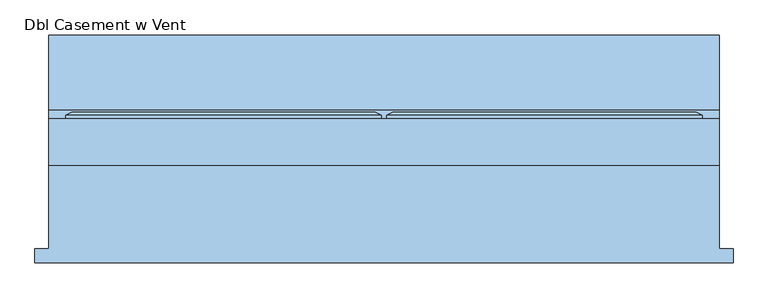
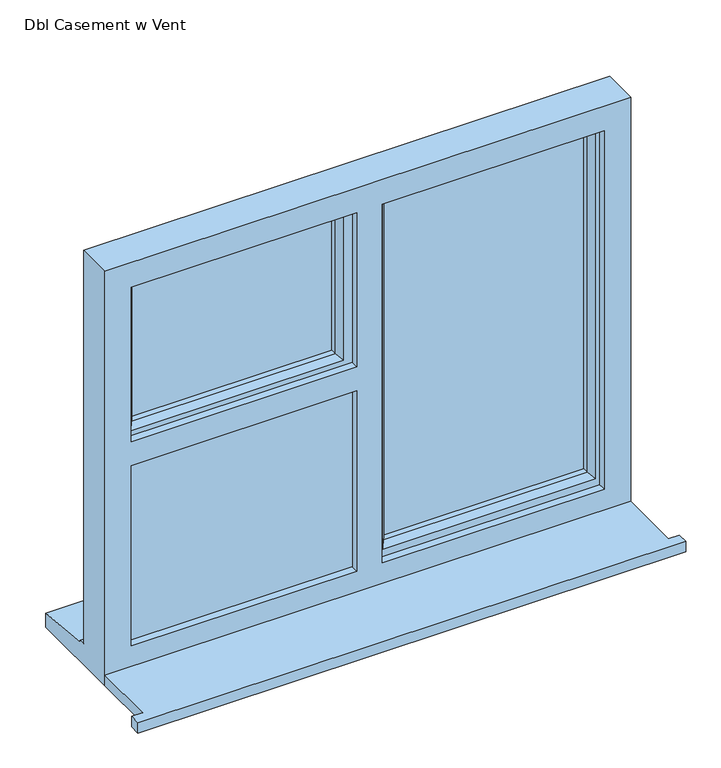
"""IFC4 building model written with IfcOpenShell, lengths in millimetres: window geometry, Dbl Casement w Vent : Doublel Casement with Vent 1200w x 1000h."""

import ifcopenshell
import ifcopenshell.guid

model = None  # the IFC model being written
_history = None  # IfcOwnerHistory: only IFC2X3 demands one
_inside = {}  # id of a spatial element -> (the spatial element, [elements in it])
_under = {}  # id of a project, library or spatial element -> (it, [spatial elements below it])
_declared = {}  # id of a project -> (the project, [libraries it declares])
_typed = {}  # id of a type object -> (the type object, [elements of that type])
_made_of = {}  # id of a material, layer set ... -> (it, [elements and type objects made of it])


def new_model(schema):
    """Start an empty IFC model of exactly this schema.

    Asked for "IFC4X3", IfcOpenShell would pick the latest addendum, in which some entities
    have other attributes; the version numbers below select the first issue.
    IFC2X3 requires an IfcOwnerHistory on every rooted entity: one is made here for all.
    """
    global model, _history
    if schema == "IFC4X3":
        model = ifcopenshell.file(schema_version=(4, 3, 0, 0))
    else:
        model = ifcopenshell.file(schema=schema)
    _inside.clear()
    _under.clear()
    _declared.clear()
    _typed.clear()
    _made_of.clear()
    _history = None
    if model.schema == "IFC2X3":
        org = make("IfcOrganization", Name="unknown")
        user = make(
            "IfcPersonAndOrganization",
            ThePerson=make("IfcPerson", FamilyName="unknown"),
            TheOrganization=org,
        )
        app = make(
            "IfcApplication",
            ApplicationDeveloper=org,
            Version="unknown",
            ApplicationFullName="unknown",
            ApplicationIdentifier="unknown",
        )
        _history = make(
            "IfcOwnerHistory",
            OwningUser=user,
            OwningApplication=app,
            ChangeAction="ADDED",
            CreationDate=0,
        )
    return model


def make(cls, **values):
    """One entity of the class cls with the attributes given. An attribute that is None is left unset."""
    return model.create_entity(
        cls, **{name: value for name, value in values.items() if value is not None}
    )


def rooted(cls, **values):
    """An entity with a GlobalId (a new one), such as an element, a storey or a relation."""
    return make(cls, GlobalId=ifcopenshell.guid.new(), OwnerHistory=_history, **values)


def si_unit(unit_type, name, prefix=None):
    """IfcSIUnit, for example si_unit("LENGTHUNIT", "METRE", prefix="MILLI")."""
    return make("IfcSIUnit", UnitType=unit_type, Prefix=prefix, Name=name)


def assignment(units):
    """IfcUnitAssignment: the units of a project."""
    return None if units is None else make("IfcUnitAssignment", Units=units)


def point(xyz):
    """IfcCartesianPoint."""
    return None if xyz is None else make("IfcCartesianPoint", Coordinates=xyz)


def direction(xyz):
    """IfcDirection."""
    return None if xyz is None else make("IfcDirection", DirectionRatios=xyz)


def frame(location, z_axis=None, x_axis=None):
    """IfcAxis2Placement3D, a coordinate frame: its origin and axes. An axis left out is left unset."""
    return make(
        "IfcAxis2Placement3D",
        Location=point(location),
        Axis=direction(z_axis),
        RefDirection=direction(x_axis),
    )


def origin():
    """The frame at (0, 0, 0) with its axes left unset."""
    return frame((0.0, 0.0, 0.0))


def place(relative_to, where):
    """IfcLocalPlacement: puts the frame where relative to a parent placement (None: the world)."""
    return make(
        "IfcLocalPlacement", PlacementRelTo=relative_to, RelativePlacement=where
    )


def context(
    kind, dimensions, precision=None, world=None, true_north=None, identifier=None
):
    """IfcGeometricRepresentationContext, for example the 3D "Model" context."""
    return make(
        "IfcGeometricRepresentationContext",
        ContextIdentifier=identifier,
        ContextType=kind,
        CoordinateSpaceDimension=dimensions,
        Precision=precision,
        WorldCoordinateSystem=world,
        TrueNorth=true_north,
    )


def project(units=None, contexts=None):
    """IfcProject with its units and contexts."""
    return rooted(
        "IfcProject",
        Name="project",
        RepresentationContexts=contexts,
        UnitsInContext=assignment(units),
    )


def spatial(cls, under=None, at=None, **own):
    """A site, building, storey or space (cls), placed at a placement, below another one or the project."""
    s = rooted(cls, ObjectPlacement=at, **own)
    if under is not None:
        _under.setdefault(under.id(), (under, []))[1].append(s)
    return s


def polyline(points):
    """IfcPolyline through the points."""
    return make("IfcPolyline", Points=[point(p) for p in points])


def outline(outer, holes=None, kind="AREA"):
    """IfcArbitraryClosedProfileDef: a profile drawn as a closed curve; with holes, ...WithVoids."""
    if holes is None:
        return make("IfcArbitraryClosedProfileDef", ProfileType=kind, OuterCurve=outer)
    return make(
        "IfcArbitraryProfileDefWithVoids",
        ProfileType=kind,
        OuterCurve=outer,
        InnerCurves=holes,
    )


def extrude(swept, where, along, depth):
    """IfcExtrudedAreaSolid: the profile swept, set in the frame where, extruded along a direction by depth."""
    return make(
        "IfcExtrudedAreaSolid",
        SweptArea=swept,
        Position=where,
        ExtrudedDirection=direction(along),
        Depth=depth,
    )


def faces_of(points, faces, orient=None, outer=None):
    """IfcFace entities. A face is a list of loops; a loop is a list of indices into points, from 0.

    orient and outer hold one flag for each loop. By default every Orientation is true, the
    first loop of a face is its IfcFaceOuterBound and the others are IfcFaceBound.
    """
    made = []
    for i, loops in enumerate(faces):
        bounds = []
        for j, loop in enumerate(loops):
            is_outer = j == 0 if outer is None else outer[i][j]
            bounds.append(
                make(
                    "IfcFaceOuterBound" if is_outer else "IfcFaceBound",
                    Bound=make("IfcPolyLoop", Polygon=[points[k] for k in loop]),
                    Orientation=True if orient is None else orient[i][j],
                )
            )
        made.append(make("IfcFace", Bounds=bounds))
    return made


def faceted_brep(points, faces, orient=None, outer=None, voids=None):
    """IfcFacetedBrep: a solid bounded by flat faces; with voids (closed shells), ...WithVoids."""
    shared = [point(p) for p in points]
    hull = make("IfcClosedShell", CfsFaces=faces_of(shared, faces, orient, outer))
    if voids is None:
        return make("IfcFacetedBrep", Outer=hull)
    return make(
        "IfcFacetedBrepWithVoids",
        Outer=hull,
        Voids=[
            make(cls, CfsFaces=faces_of(shared, fs, o, b)) for cls, fs, o, b in voids
        ],
    )


def shape(context_of_items, identifier, shape_type, items):
    """IfcShapeRepresentation: the items that make up one representation, for example the "Body"."""
    return make(
        "IfcShapeRepresentation",
        ContextOfItems=context_of_items,
        RepresentationIdentifier=identifier,
        RepresentationType=shape_type,
        Items=items,
    )


def source(mapping_origin, context_of_items, identifier, shape_type, items):
    """IfcRepresentationMap: a shape defined once, which mapped items show again and again."""
    return make(
        "IfcRepresentationMap",
        MappingOrigin=mapping_origin,
        MappedRepresentation=shape(context_of_items, identifier, shape_type, items),
    )


def transform(
    local_origin,
    x_axis=None,
    y_axis=None,
    z_axis=None,
    scale=None,
    scale2=None,
    scale3=None,
    uniform=True,
):
    """IfcCartesianTransformationOperator3D, or its non-uniform kind. x_axis, y_axis, z_axis: its Axis1, 2, 3."""
    if uniform:
        return make(
            "IfcCartesianTransformationOperator3D",
            Axis1=direction(x_axis),
            Axis2=direction(y_axis),
            LocalOrigin=point(local_origin),
            Scale=scale,
            Axis3=direction(z_axis),
        )
    return make(
        "IfcCartesianTransformationOperator3DnonUniform",
        Axis1=direction(x_axis),
        Axis2=direction(y_axis),
        LocalOrigin=point(local_origin),
        Scale=scale,
        Axis3=direction(z_axis),
        Scale2=scale2,
        Scale3=scale3,
    )


def mapped(mapping_source, mapping_target):
    """IfcMappedItem: shows the shape of a source again, moved by a transform."""
    return make(
        "IfcMappedItem", MappingSource=mapping_source, MappingTarget=mapping_target
    )


def made_of(thing, what):
    """Note that an element or type object is made of a material, layer set ...; save() writes the relation."""
    if what is not None:
        _made_of.setdefault(what.id(), (what, []))[1].append(thing)
    return thing


def element(
    cls,
    number,
    at=None,
    inside=None,
    cuts=None,
    type_object=None,
    material=None,
    context=None,
    identifier="Body",
    shape_type=None,
    held_by="IfcProductDefinitionShape",
    body=None,
    shapes=None,
    **own,
):
    """One element of the class cls, such as IfcWall. Its Tag is "e" and its number.

    at: its placement. inside: the storey or other place that contains it. cuts: it is an
    opening in that element (IfcRelVoidsElement). A single representation is given by context,
    identifier, shape_type and body (its items); several are given by shapes. held_by: the class
    of the entity that holds the representations. save() writes the other relations.
    """
    e = rooted(cls, Tag="e%d" % number, ObjectPlacement=at, **own)
    if body is not None:
        shapes = [shape(context, identifier, shape_type, body)]
    if shapes is not None:
        e.Representation = make(held_by, Representations=shapes)
    if inside is not None:
        _inside.setdefault(inside.id(), (inside, []))[1].append(e)
    if cuts is not None:
        rooted(
            "IfcRelVoidsElement", RelatingBuildingElement=cuts, RelatedOpeningElement=e
        )
    if type_object is not None:
        _typed.setdefault(type_object.id(), (type_object, []))[1].append(e)
    return made_of(e, material)


def aggregate(whole, parts):
    """IfcRelAggregates: a whole, such as a stair, and the parts it consists of."""
    return rooted("IfcRelAggregates", RelatingObject=whole, RelatedObjects=parts)


def save(model, path):
    """Write the relations noted so far, then the file.

    IfcRelAggregates (storeys below a building ...), IfcRelContainedInSpatialStructure (elements
    in a storey), IfcRelDefinesByType, IfcRelAssociatesMaterial and IfcRelDeclares: one each for
    every whole, place, type object, material and project.
    """
    for whole, parts in _under.values():
        aggregate(whole, parts)
    for where, things in _inside.values():
        rooted(
            "IfcRelContainedInSpatialStructure",
            RelatedElements=things,
            RelatingStructure=where,
        )
    for kind, things in _typed.values():
        rooted("IfcRelDefinesByType", RelatedObjects=things, RelatingType=kind)
    for what, things in _made_of.values():
        rooted("IfcRelAssociatesMaterial", RelatedObjects=things, RelatingMaterial=what)
    for by, libraries in _declared.values():
        rooted("IfcRelDeclares", RelatingContext=by, RelatedDefinitions=libraries)
    model.write(path)


def dbl_casement_w_vent_67fd5172(model_context):
    return source(origin(), model_context, "Body", "SolidModel", [
        extrude(outline(polyline([(-910.0, -182.7934322), (-910.0, -157.7934322), (-885.0, -157.7934322), (-885.0, -8.2934322), (315.0, -8.2934322), (315.0, -157.7934322), (340.0, -157.7934322), (340.0, -182.7934322), (-910.0, -182.7934322)])), frame((0.0, 0.0, 1110.0), z_axis=(0.0, 0.0, 1.0), x_axis=(1.0, 0.0, 0.0)), (0.0, 0.0, 1.0), 25.0),
        faceted_brep([(-855.0, 74.7065678, 2080.0), (-855.0, 80.4800705, 2080.0), (-855.0, 80.4800705, 1650.0), (-855.0, 74.7065678, 1650.0), (-845.0, 9.7065678, 2070.0), (-845.0, 74.7065678, 2070.0), (-845.0, 74.7065678, 1660.0), (-845.0, 9.7065678, 1660.0), (-805.0, 24.1994677, 2030.0), (-815.1480377, 9.7065678, 2040.1480377), (-815.1480377, 9.7065678, 1689.8519623), (-805.0, 24.1994677, 1700.0), (-805.0, 38.7065678, 2030.0), (-805.0, 38.7065678, 1700.0), (-815.0, 62.7065678, 2040.0), (-815.0, 38.7065678, 2040.0), (-815.0, 38.7065678, 1690.0), (-815.0, 62.7065678, 1690.0), (-805.0, 80.4800705, 2030.0), (-805.0, 62.7065678, 2030.0), (-805.0, 62.7065678, 1700.0), (-805.0, 80.4800705, 1700.0), (-822.4457548, 86.2535732, 2047.4457548), (-822.4457548, 86.2535732, 1682.5542452), (-844.2153903, 86.2535732, 2069.2153903), (-844.2153903, 86.2535732, 1660.7846097), (-290.0, 80.4800705, 1650.0), (-290.0, 74.7065678, 1650.0), (-300.0, 74.7065678, 1660.0), (-300.0, 9.7065678, 1660.0), (-329.8519623, 9.7065678, 1689.8519623), (-340.0, 24.1994677, 1700.0), (-340.0, 38.7065678, 1700.0), (-330.0, 38.7065678, 1690.0), (-330.0, 62.7065678, 1690.0), (-340.0, 62.7065678, 1700.0), (-340.0, 80.4800705, 1700.0), (-322.5542452, 86.2535732, 1682.5542452), (-300.7846097, 86.2535732, 1660.7846097), (-290.0, 80.4800705, 2080.0), (-290.0, 74.7065678, 2080.0), (-300.0, 74.7065678, 2070.0), (-300.0, 9.7065678, 2070.0), (-329.8519623, 9.7065678, 2040.1480377), (-340.0, 24.1994677, 2030.0), (-340.0, 38.7065678, 2030.0), (-330.0, 38.7065678, 2040.0), (-330.0, 62.7065678, 2040.0), (-340.0, 62.7065678, 2030.0), (-340.0, 80.4800705, 2030.0), (-322.5542452, 86.2535732, 2047.4457548), (-300.7846097, 86.2535732, 2069.2153903)], [[[0, 1, 2, 3]], [[4, 5, 6, 7]], [[8, 9, 10, 11]], [[12, 8, 11, 13]], [[14, 15, 16, 17]], [[18, 19, 20, 21]], [[22, 18, 21, 23]], [[1, 24, 25, 2]], [[3, 2, 26, 27]], [[7, 6, 28, 29]], [[11, 10, 30, 31]], [[13, 11, 31, 32]], [[17, 16, 33, 34]], [[21, 20, 35, 36]], [[23, 21, 36, 37]], [[2, 25, 38, 26]], [[27, 26, 39, 40]], [[29, 28, 41, 42]], [[31, 30, 43, 44]], [[32, 31, 44, 45]], [[34, 33, 46, 47]], [[36, 35, 48, 49]], [[37, 36, 49, 50]], [[26, 38, 51, 39]], [[40, 39, 1, 0]], [[3, 27, 40, 0], [5, 41, 28, 6]], [[42, 41, 5, 4]], [[7, 29, 42, 4], [9, 43, 30, 10]], [[44, 43, 9, 8]], [[45, 44, 8, 12]], [[15, 46, 33, 16], [13, 32, 45, 12]], [[47, 46, 15, 14]], [[17, 34, 47, 14], [19, 48, 35, 20]], [[49, 48, 19, 18]], [[50, 49, 18, 22]], [[24, 51, 38, 25], [23, 37, 50, 22]], [[39, 51, 24, 1]]]),
        extrude(outline(polyline([(245.0, 38.7065678), (-240.0, 38.7065678), (-240.0, 62.7065678), (245.0, 62.7065678), (245.0, 38.7065678)])), frame((0.0, 0.0, 1203.0), z_axis=(0.0, 0.0, 1.0), x_axis=(1.0, 0.0, 0.0)), (0.0, 0.0, 1.0), 837.0),
        extrude(outline(polyline([(-330.0, 38.7065678), (-815.0, 38.7065678), (-815.0, 62.7065678), (-330.0, 62.7065678), (-330.0, 38.7065678)])), frame((0.0, 0.0, 1690.0), z_axis=(0.0, 0.0, 1.0), x_axis=(1.0, 0.0, 0.0)), (0.0, 0.0, 1.0), 350.0),
        extrude(outline(polyline([(-845.0, 33.7065678), (-300.0, 33.7065678), (-300.0, 9.7065678), (-845.0, 9.7065678), (-845.0, 33.7065678)])), frame((0.0, 0.0, 1173.0), z_axis=(0.0, 0.0, 1.0), x_axis=(1.0, 0.0, 0.0)), (0.0, 0.0, 1.0), 457.0),
        faceted_brep([(315.0, -8.2934322, 2110.0), (-885.0, -8.2934322, 2110.0), (-885.0, -8.2934322, 1110.0), (315.0, -8.2934322, 1110.0), (-825.0, -8.2934322, 1185.0), (-825.0, -8.2934322, 1620.0), (-310.0, -8.2934322, 1620.0), (-310.0, -8.2934322, 1185.0), (-825.0, -8.2934322, 2050.0), (-310.0, -8.2934322, 2050.0), (-310.0, -8.2934322, 1678.0), (-825.0, -8.2934322, 1678.0), (-252.0, -8.2934322, 2050.0), (255.0, -8.2934322, 2050.0), (255.0, -8.2934322, 1185.0), (-252.0, -8.2934322, 1185.0), (-885.0, 74.7065678, 2110.0), (-885.0, 74.7065678, 1161.0), (-885.0, 89.7065678, 1159.68767), (-885.0, 89.7065678, 1154.7449676), (-885.0, 224.7065678, 1143.8088847), (-885.0, 224.7065678, 1110.0), (315.0, 74.7065678, 2110.0), (315.0, 74.7065678, 1161.0), (-310.0, 74.7065678, 1173.0), (-310.0, 74.7065678, 1620.0), (-845.0, 74.7065678, 1620.0), (-845.0, 74.7065678, 1173.0), (-310.0, 74.7065678, 2070.0), (-845.0, 74.7065678, 2070.0), (-845.0, 74.7065678, 1660.0), (-310.0, 74.7065678, 1660.0), (275.0, 74.7065678, 1173.0), (275.0, 74.7065678, 2070.0), (-270.0, 74.7065678, 2070.0), (-270.0, 74.7065678, 1173.0), (-845.0, 9.7065678, 2070.0), (-845.0, 9.7065678, 1660.0), (-845.0, 9.7065678, 1630.0), (-845.0, 9.7065678, 1173.0), (-845.0, 33.7065678, 1620.0), (-845.0, 33.7065678, 1630.0), (-300.0, 9.7065678, 2070.0), (-300.0, 9.7065678, 1660.0), (-310.0, 9.7065678, 2050.0), (-825.0, 9.7065678, 2050.0), (-825.0, 9.7065678, 1678.0), (-310.0, 9.7065678, 1678.0), (-270.0, 9.7065678, 2070.0), (275.0, 9.7065678, 2070.0), (275.0, 9.7065678, 1173.0), (-270.0, 9.7065678, 1173.0), (255.0, 9.7065678, 2050.0), (-252.0, 9.7065678, 2050.0), (-252.0, 9.7065678, 1185.0), (255.0, 9.7065678, 1185.0), (-300.0, 9.7065678, 1173.0), (-300.0, 9.7065678, 1630.0), (-825.0, 9.7065678, 1185.0), (-310.0, 9.7065678, 1185.0), (-310.0, 9.7065678, 1620.0), (-825.0, 9.7065678, 1620.0), (-310.0, 33.7065678, 2070.0), (-300.0, 33.7065678, 2070.0), (315.0, 224.7065678, 1110.0), (315.0, 224.7065678, 1143.8088847), (315.0, 89.7065678, 1154.7449676), (315.0, 89.7065678, 1159.68767), (-300.0, 33.7065678, 1660.0), (-300.0, 33.7065678, 1630.0), (-300.0, 33.7065678, 1173.0), (-310.0, 33.7065678, 1660.0), (-310.0, 33.7065678, 1173.0), (-310.0, 33.7065678, 1620.0)], [[[0, 1, 2, 3], [4, 5, 6, 7], [8, 9, 10, 11], [12, 13, 14, 15]], [[1, 16, 17, 18, 19, 20, 21, 2]], [[16, 22, 23, 17], [24, 25, 26, 27], [28, 29, 30, 31], [32, 33, 34, 35]], [[29, 36, 37, 30]], [[38, 39, 27, 26, 40, 41]], [[36, 42, 43, 37], [44, 45, 46, 47]], [[48, 49, 50, 51], [52, 53, 54, 55]], [[56, 39, 38, 57], [58, 59, 60, 61]], [[45, 8, 11, 46]], [[4, 58, 61, 5]], [[1, 0, 22, 16]], [[36, 29, 28, 62, 63, 42]], [[33, 49, 48, 34]], [[8, 45, 44, 9]], [[52, 13, 12, 53]], [[22, 0, 3, 64, 65, 66, 67, 23]], [[33, 32, 50, 49]], [[13, 52, 55, 14]], [[43, 42, 63, 68]], [[69, 70, 56, 57]], [[63, 62, 71, 68]], [[72, 70, 69, 41, 40, 73]], [[62, 28, 31, 71]], [[24, 72, 73, 25]], [[35, 34, 48, 51]], [[53, 12, 15, 54]], [[9, 44, 47, 10]], [[59, 7, 6, 60]], [[64, 3, 2, 21]], [[65, 64, 21, 20]], [[66, 65, 20, 19]], [[67, 66, 19, 18]], [[23, 67, 18, 17]], [[24, 27, 39, 56, 70, 72]], [[32, 35, 51, 50]], [[15, 14, 55, 54]], [[59, 58, 4, 7]], [[57, 38, 41, 69]], [[26, 25, 73, 40]], [[31, 30, 37, 43, 68, 71]], [[47, 46, 11, 10]], [[61, 60, 6, 5]]]),
        extrude(outline(polyline([(1660.0, -825.0), (1660.0, -845.0), (1173.0, -845.0), (1173.0, -310.0), (1193.0, -310.0), (1193.0, -825.0), (1660.0, -825.0)])), frame((0.0, 33.7065678, 0.0), z_axis=(0.0, 1.0, 0.0), x_axis=(0.0, 0.0, 1.0)), (0.0, 0.0, 1.0), 41.0),
        faceted_brep([(-280.0, 74.7065678, 2080.0), (-280.0, 80.4800705, 2080.0), (-280.0, 80.4800705, 1163.0), (-280.0, 74.7065678, 1163.0), (-270.0, 9.7065678, 2070.0), (-270.0, 74.7065678, 2070.0), (-270.0, 74.7065678, 1173.0), (-270.0, 9.7065678, 1173.0), (-230.0, 24.1994677, 2030.0), (-240.1480377, 9.7065678, 2040.1480377), (-240.1480377, 9.7065678, 1202.8519623), (-230.0, 24.1994677, 1213.0), (-230.0, 38.7065678, 2030.0), (-230.0, 38.7065678, 1213.0), (-240.0, 62.7065678, 2040.0), (-240.0, 38.7065678, 2040.0), (-240.0, 38.7065678, 1203.0), (-240.0, 62.7065678, 1203.0), (-230.0, 80.4800705, 2030.0), (-230.0, 62.7065678, 2030.0), (-230.0, 62.7065678, 1213.0), (-230.0, 80.4800705, 1213.0), (-247.4457548, 86.2535732, 2047.4457548), (-247.4457548, 86.2535732, 1195.5542452), (-269.2153903, 86.2535732, 2069.2153903), (-269.2153903, 86.2535732, 1173.7846097), (285.0, 80.4800705, 1163.0), (285.0, 74.7065678, 1163.0), (275.0, 74.7065678, 1173.0), (275.0, 9.7065678, 1173.0), (245.1480377, 9.7065678, 1202.8519623), (235.0, 24.1994677, 1213.0), (235.0, 38.7065678, 1213.0), (245.0, 38.7065678, 1203.0), (245.0, 62.7065678, 1203.0), (235.0, 62.7065678, 1213.0), (235.0, 80.4800705, 1213.0), (252.4457548, 86.2535732, 1195.5542452), (274.2153903, 86.2535732, 1173.7846097), (285.0, 80.4800705, 2080.0), (285.0, 74.7065678, 2080.0), (275.0, 74.7065678, 2070.0), (275.0, 9.7065678, 2070.0), (245.1480377, 9.7065678, 2040.1480377), (235.0, 24.1994677, 2030.0), (235.0, 38.7065678, 2030.0), (245.0, 38.7065678, 2040.0), (245.0, 62.7065678, 2040.0), (235.0, 62.7065678, 2030.0), (235.0, 80.4800705, 2030.0), (252.4457548, 86.2535732, 2047.4457548), (274.2153903, 86.2535732, 2069.2153903)], [[[0, 1, 2, 3]], [[4, 5, 6, 7]], [[8, 9, 10, 11]], [[12, 8, 11, 13]], [[14, 15, 16, 17]], [[18, 19, 20, 21]], [[22, 18, 21, 23]], [[1, 24, 25, 2]], [[3, 2, 26, 27]], [[7, 6, 28, 29]], [[11, 10, 30, 31]], [[13, 11, 31, 32]], [[17, 16, 33, 34]], [[21, 20, 35, 36]], [[23, 21, 36, 37]], [[2, 25, 38, 26]], [[27, 26, 39, 40]], [[29, 28, 41, 42]], [[31, 30, 43, 44]], [[32, 31, 44, 45]], [[34, 33, 46, 47]], [[36, 35, 48, 49]], [[37, 36, 49, 50]], [[26, 38, 51, 39]], [[40, 39, 1, 0]], [[3, 27, 40, 0], [5, 41, 28, 6]], [[42, 41, 5, 4]], [[7, 29, 42, 4], [9, 43, 30, 10]], [[44, 43, 9, 8]], [[45, 44, 8, 12]], [[15, 46, 33, 16], [13, 32, 45, 12]], [[47, 46, 15, 14]], [[17, 34, 47, 14], [19, 48, 35, 20]], [[49, 48, 19, 18]], [[50, 49, 18, 22]], [[24, 51, 38, 25], [23, 37, 50, 22]], [[39, 51, 24, 1]]]),
    ])


if __name__ == "__main__":
    model = new_model("IFC4")
    model_context = context("Model", 3, world=origin())
    ifc_project = project(units=[si_unit("LENGTHUNIT", "METRE", prefix="MILLI")], contexts=[model_context])
    site = spatial("IfcSite", under=ifc_project)
    building = spatial("IfcBuilding", under=site)
    placement = place(None, origin())
    dbl_casement_w_vent_shape = dbl_casement_w_vent_67fd5172(model_context)
    element("IfcWindow", 1, ObjectType="Dbl Casement w Vent : Doublel Casement with Vent 1200w x 1000h", at=placement, inside=building, context=model_context, shape_type="MappedRepresentation", body=[
        mapped(dbl_casement_w_vent_shape, transform((0.0, 0.0, 0.0), x_axis=(1.0, 0.0, 0.0), y_axis=(0.0, 1.0, 0.0), z_axis=(0.0, 0.0, 1.0))),
    ])
    save(model, "model.ifc")

# Revit data of these elements
# Type "Dbl Casement w Vent : Doublel Casement with Vent 1200w x 1000h"
#   Description = "Double Casement Window with Opening Sash Vents"
#   Type Mark = "45"
#   Operation = "TriplePanelRight"
#   Construction Type Id = "GSP4R"
#   Manufacturer = "Revit"
#   Keynote = "L10"
#   Analytic Construction = "1/8 in Pilkington single glazing"
#   Wrap Layers (Ext) from Ext = 102.5 mm
#   Wrap Layers (Int) from Ext = 177.5 mm
#   Window Board Projection = 25 mm
#   Window Board Extension = 25 mm
#   Visual Light Transmittance = 0.9
#   Vent Depth = 450 mm
#   Thermal Resistance (R) = 0.271106 (m²·K)/W
#   Solar Heat Gain Coefficient = 0.78
#   Rough Width = 1200 mm
#   Rough Height = 1000 mm
#   Frame Height = 1350 mm
#   Height = 1000 mm
#   Width = 1200 mm
#   Heat Transfer Coefficient (U) = 3.6886 W/(m²·K)
#   Glazing Thickness = 24 mm
#   FrameOffset - External = 100 mm
#   Frame Depth = 65 mm
#   Default Head Height = 2110 mm
#   Cill Depth = 150 mm
#   Cavity Closer Width = 75 mm
#   Cavity Closer Offset from Ext = 110 mm
#   Cavity Closer Depth = 105 mm
#   Vis - Cavity Closers = yes
#   Define Thermal Properties by = 1
#   Material Trim = Window Frame
#   Material Glass = Glass
#   Material Frame = Window Frame
#   Wall Closure = (empty or 0)
# Element 1 (IfcWindow, "Dbl Casement w Vent : Doublel Casement with Vent 1200w x 1000h")
#   Materials on its faces: "Window Frame", "Glass"
# Materials
#   "Window Frame": class "Miscellaneous", colour RGB 249 249 249, transparency 0, Keynote = "L10"
#   "Glass": class "Glass", colour RGB 0 128 192, transparency 0.9, Description = "Soda Lime Glass", Cost = 0
